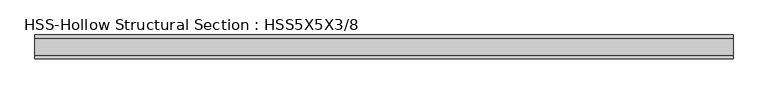
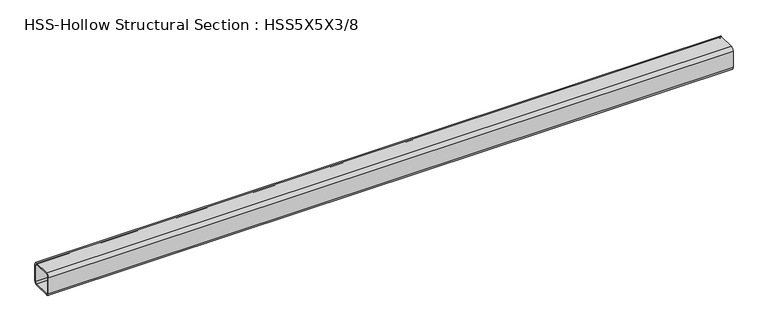
"""IFC4 building model written with IfcOpenShell, lengths in millimetres: member geometry, HSS-Hollow Structural Section : HSS5X5X3/8."""

from ifc_helpers import new_model, si_unit, point, frame, frame_2d, origin, place, context, project, spatial, polyline, circle_curve, trimmed, segment, composite_curve, outline, extrude, source, transform, mapped, element, save


def hss_hollow_structural_section_hss5x5x3_8_db42e5ad(model_context):
    return source(origin(), model_context, "Body", "SweptSolid", [
        extrude(outline(composite_curve([segment(polyline([(63.5, 45.7708), (63.5, -45.7708)]), True, "CONTINUOUS"), segment(trimmed(circle_curve(frame_2d((45.7708, -45.7708)), 17.7292), [point((63.5, -45.7708))], [point((45.7708, -63.5))], False, "CARTESIAN"), True, "CONTINUOUS"), segment(polyline([(45.7708, -63.5), (-45.7708, -63.5)]), True, "CONTINUOUS"), segment(trimmed(circle_curve(frame_2d((-45.7708, -45.7708)), 17.7292), [point((-45.7708, -63.5))], [point((-63.5, -45.7708))], False, "CARTESIAN"), True, "CONTINUOUS"), segment(polyline([(-63.5, -45.7708), (-63.5, 45.7708)]), True, "CONTINUOUS"), segment(trimmed(circle_curve(frame_2d((-45.7708, 45.7708)), 17.7292), [point((-63.5, 45.7708))], [point((-45.7708, 63.5))], False, "CARTESIAN"), True, "CONTINUOUS"), segment(polyline([(-45.7708, 63.5), (45.7708, 63.5)]), True, "CONTINUOUS"), segment(trimmed(circle_curve(frame_2d((45.7708, 45.7708)), 17.7292), [point((45.7708, 63.5))], [point((63.5, 45.7708))], False, "CARTESIAN"), True, "CONTINUOUS")], self_intersect=False), holes=[composite_curve([segment(trimmed(circle_curve(frame_2d((-45.7708, 45.7708)), 8.8646), [point((-45.7708, 54.6354))], [point((-54.6354, 45.7708))], True, "CARTESIAN"), True, "CONTINUOUS"), segment(polyline([(-54.6354, 45.7708), (-54.6354, -45.7708)]), True, "CONTINUOUS"), segment(trimmed(circle_curve(frame_2d((-45.7708, -45.7708)), 8.8646), [point((-54.6354, -45.7708))], [point((-45.7708, -54.6354))], True, "CARTESIAN"), True, "CONTINUOUS"), segment(polyline([(-45.7708, -54.6354), (45.7708, -54.6354)]), True, "CONTINUOUS"), segment(trimmed(circle_curve(frame_2d((45.7708, -45.7708)), 8.8646), [point((45.7708, -54.6354))], [point((54.6354, -45.7708))], True, "CARTESIAN"), True, "CONTINUOUS"), segment(polyline([(54.6354, -45.7708), (54.6354, 45.7708)]), True, "CONTINUOUS"), segment(trimmed(circle_curve(frame_2d((45.7708, 45.7708)), 8.8646), [point((54.6354, 45.7708))], [point((45.7708, 54.6354))], True, "CARTESIAN"), True, "CONTINUOUS"), segment(polyline([(45.7708, 54.6354), (-45.7708, 54.6354)]), True, "CONTINUOUS")], self_intersect=False)]), frame((-1936.5194771, 0.0, 0.0), z_axis=(1.0, 0.0, 0.0), x_axis=(0.0, 1.0, 0.0)), (0.0, 0.0, 1.0), 3709.3028173),
    ])


if __name__ == "__main__":
    model = new_model("IFC4")
    model_context = context("Model", 3, world=origin())
    ifc_project = project(units=[si_unit("LENGTHUNIT", "METRE", prefix="MILLI")], contexts=[model_context])
    site = spatial("IfcSite", under=ifc_project)
    building = spatial("IfcBuilding", under=site)
    placement = place(None, origin())
    hss_hollow_structural_section_hss5x5x3_8_shape = hss_hollow_structural_section_hss5x5x3_8_db42e5ad(model_context)
    element("IfcMember", 1, ObjectType="HSS-Hollow Structural Section : HSS5X5X3/8", at=placement, inside=building, context=model_context, shape_type="MappedRepresentation", body=[
        mapped(hss_hollow_structural_section_hss5x5x3_8_shape, transform((0.0, 0.0, 0.0), x_axis=(1.0, 0.0, 0.0), y_axis=(0.0, 1.0, 0.0), z_axis=(0.0, 0.0, 1.0))),
    ])
    save(model, "model.ifc")

# Revit data of these elements
# Type "HSS-Hollow Structural Section : HSS5X5X3/8"
#   Assembly Code = "B10"
#   Shape = "Square"
#   W = 22.3
#   Ht = 0' - 5"
#   Length [instance default] = 5' - 0"
#   b = 0' - 5"
#   kr = 0' - 0.698"
#   t = 0' - 0.349"
#   A = 0.0429167 SF
#   Structural Material [instance default] = Steel ASTM A500, Grade B, Rectangular and Square
# Element 1 (IfcMember, "HSS-Hollow Structural Section : HSS5X5X3/8")
#   Materials on its faces: "Steel ASTM A500, Grade B, Rectangular and Square"
# Materials
#   "Steel ASTM A500, Grade B, Rectangular and Square": class "Metal", colour RGB 199 199 199, transparency 0, Description = "Carbon steel", Cost = 0
